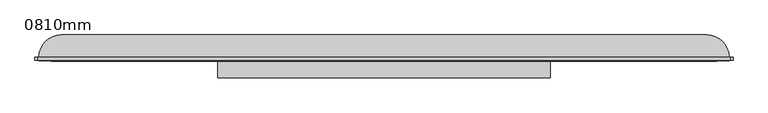
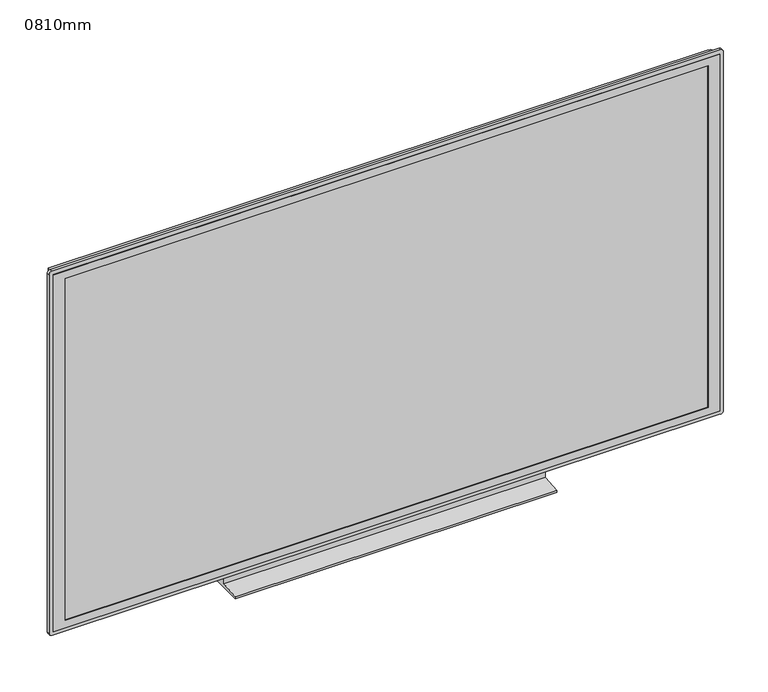
"""IFC4 building model written with IfcOpenShell, lengths in millimetres: furniture geometry, M_TV - Flat Screen : 0810mm."""

from ifc_helpers import new_model, si_unit, point, frame, frame_2d, origin, place, context, project, spatial, polyline, circle_curve, ellipse_curve, trimmed, segment, composite_curve, outline, extrude, faceted_brep, source, transform, mapped, element, save
from ifc_brep_helpers import plane_surface, cylinder_surface, advanced_brep


def furniture_0810mm_1eea789d(model_context):
    return source(origin(), model_context, "Body", "SolidModel", [
        advanced_brep(
        [(-1698.1126034, -51.4613764, 80.0), (1690.2235751, -51.4613764, 80.0), (1690.2235751, -51.4613764, 1998.6077952), (-1698.1126034, -51.4613764, 1998.6077952), (1580.2235751, 58.5386236, 80.0), (-1588.1126034, 58.5386236, 80.0), (-1588.1126034, 58.5386236, 1888.6077952), (1580.2235751, 58.5386236, 1888.6077952)],
        [
            (0, 1),
            (1, 2),
            (2, 3),
            (3, 0),
            (4, 5),
            (5, 6),
            (6, 7),
            (7, 4),
            (0, 5, circle_curve(frame((-1588.1126034, -51.4613764, 80.0), z_axis=(0.0, 0.0, -1.0), x_axis=(-1.0, 0.0, 0.0)), 110.0)),
            (4, 1, circle_curve(frame((1580.2235751, -51.4613764, 80.0), z_axis=(0.0, 0.0, -1.0), x_axis=(1.0, 0.0, 0.0)), 110.0)),
            (7, 2, ellipse_curve(frame((1580.2235751, -51.4613764, 1888.6077952), z_axis=(0.7071067811865475, 0.0, -0.7071067811865475), x_axis=(0.7071067811865474, 0.0, 0.7071067811865476)), 155.5634919, 110.0)),
            (6, 3, ellipse_curve(frame((-1588.1126034, -51.4613764, 1888.6077952), z_axis=(0.7071067811865475, 0.0, 0.7071067811865475), x_axis=(-0.7071067811865476, 0.0, 0.7071067811865474)), 155.5634919, 110.0)),
        ],
        [
            plane_surface(frame((-1698.1126034, -51.4613764, 1998.6077952), z_axis=(0.0, -1.0, 0.0), x_axis=(-1.0, 0.0, 0.0))),
            plane_surface(frame((-1698.1126034, 58.5386236, 1998.6077952), z_axis=(0.0, 1.0, 0.0), x_axis=(1.0, 0.0, 0.0))),
            plane_surface(frame((-1698.1126034, -51.4613764, 80.0), z_axis=(0.0, 0.0, -1.0), x_axis=(0.0, 1.0, 0.0))),
            cylinder_surface(frame((1580.2235751, -51.4613764, 80.0), z_axis=(0.0, 0.0, 1.0), x_axis=(1.0, 0.0, 0.0)), 110.0),
            cylinder_surface(frame((1690.2235751, -51.4613764, 1888.6077952), z_axis=(-1.0, 0.0, 0.0), x_axis=(0.0, 0.0, 1.0)), 110.0),
            cylinder_surface(frame((-1588.1126034, -51.4613764, 1998.6077952), z_axis=(0.0, 0.0, -1.0), x_axis=(-1.0, 0.0, 0.0)), 110.0),
        ],
        [
            (0, [[1, 2, 3, 4]]),
            (1, [[5, 6, 7, 8]]),
            (2, [[-1, 9, -5, 10]]),
            (3, [[11, -2, -10, -8]]),
            (4, [[-11, -7, 12, -3]]),
            (5, [[-12, -6, -9, -4]]),
        ],
    ),
        extrude(outline(composite_curve([segment(polyline([(2018.6077952, 1695.2235751), (2018.6077952, -1703.1126034)]), True, "CONTINUOUS"), segment(trimmed(circle_curve(frame_2d((2003.6077952, -1703.1126034)), 15.0), [point((2018.6077952, -1703.1126034))], [point((2003.6077952, -1718.1126034))], False, "CARTESIAN"), True, "CONTINUOUS"), segment(polyline([(2003.6077952, -1718.1126034), (75.0, -1718.1126034)]), True, "CONTINUOUS"), segment(trimmed(circle_curve(frame_2d((75.0, -1703.1126034)), 15.0), [point((75.0, -1718.1126034))], [point((60.0, -1703.1126034))], False, "CARTESIAN"), True, "CONTINUOUS"), segment(polyline([(60.0, -1703.1126034), (60.0, 1695.2235751)]), True, "CONTINUOUS"), segment(trimmed(circle_curve(frame_2d((75.0, 1695.2235751)), 15.0), [point((60.0, 1695.2235751))], [point((75.0, 1710.2235751))], False, "CARTESIAN"), True, "CONTINUOUS"), segment(polyline([(75.0, 1710.2235751), (2003.6077952, 1710.2235751)]), True, "CONTINUOUS"), segment(trimmed(circle_curve(frame_2d((2003.6077952, 1695.2235751)), 15.0), [point((2003.6077952, 1710.2235751))], [point((2018.6077952, 1695.2235751))], False, "CARTESIAN"), True, "CONTINUOUS")], self_intersect=False), holes=[polyline([(1998.6077952, 1690.2235751), (80.0, 1690.2235751), (80.0, -1698.1126034), (1998.6077952, -1698.1126034), (1998.6077952, 1690.2235751)])]), frame((0.0, -66.4613764, 0.0), z_axis=(0.0, 1.0, 0.0), x_axis=(0.0, 0.0, 1.0)), (0.0, 0.0, 1.0), 15.0),
        faceted_brep([(1690.2235751, -69.4613764, 1998.6077952), (-1698.1126034, -69.4613764, 1998.6077952), (-1698.1126034, -69.4613764, 80.0), (1690.2235751, -69.4613764, 80.0), (-1638.1126034, -69.4613764, 1958.6077952), (1630.2235751, -69.4613764, 1958.6077952), (1630.2235751, -69.4613764, 120.0), (-1638.1126034, -69.4613764, 120.0), (1690.2235751, -51.4613764, 1998.6077952), (1690.2235751, -51.4613764, 80.0), (-1698.1126034, -51.4613764, 80.0), (-1698.1126034, -51.4613764, 1998.6077952), (-1638.1126034, -66.4613764, 1958.6077952), (-1638.1126034, -66.4613764, 120.0), (1630.2235751, -66.4613764, 120.0), (1630.2235751, -66.4613764, 1958.6077952)], [[[0, 1, 2, 3], [4, 5, 6, 7]], [[8, 9, 10, 11]], [[1, 0, 8, 11]], [[2, 1, 11, 10]], [[3, 2, 10, 9]], [[0, 3, 9, 8]], [[12, 13, 14, 15]], [[12, 15, 5, 4]], [[15, 14, 6, 5]], [[14, 13, 7, 6]], [[13, 12, 4, 7]]]),
        extrude(outline(polyline([(-51.4613764, 80.0), (-1.4613764, 80.0), (48.5386236, 0.0), (-151.4613764, 0.0), (-151.4613764, 10.0), (-51.4613764, 20.0), (-51.4613764, 80.0)])), frame((-821.0285588, 0.0, 0.0), z_axis=(1.0, 0.0, 0.0), x_axis=(0.0, 1.0, 0.0)), (0.0, 0.0, 1.0), 1634.1680892),
    ])


if __name__ == "__main__":
    model = new_model("IFC4")
    model_context = context("Model", 3, world=origin())
    ifc_project = project(units=[si_unit("LENGTHUNIT", "METRE", prefix="MILLI")], contexts=[model_context])
    site = spatial("IfcSite", under=ifc_project)
    building = spatial("IfcBuilding", under=site)
    placement = place(None, origin())
    furniture_0810mm_shape = furniture_0810mm_1eea789d(model_context)
    element("IfcFurniture", 1, ObjectType="M_TV - Flat Screen : 0810mm", at=placement, inside=building, context=model_context, shape_type="MappedRepresentation", body=[
        mapped(furniture_0810mm_shape, transform((0.0, 0.0, 0.0), x_axis=(1.0, 0.0, 0.0), y_axis=(0.0, 1.0, 0.0), z_axis=(0.0, 0.0, 1.0))),
    ])
    save(model, "model.ifc")

# Revit data of these elements
# Type "M_TV - Flat Screen : 0810mm"
#   SinAng = 0.49 mm
#   L = 3268.336 mm
#   H = 1838.608 mm
#   Thickness = 110 mm
#   Diagonal = 3750 mm
#   CosAng = 0.872 mm
#   Stand [instance default] = yes
#   Default Elevation = 0
# Element 1 (IfcFurniture, "M_TV - Flat Screen : 0810mm")
#   Materials on its faces: "TV - Black", "TV - Glass", "TV - Screen"
# Materials
#   "TV - Black": class "Miscellaneous", colour RGB 49 49 49, transparency 0
#   "TV - Glass": class "Miscellaneous", colour RGB 157 157 157, transparency 0.9
#   "TV - Screen": class "Miscellaneous", colour RGB 0 0 0, transparency 0
